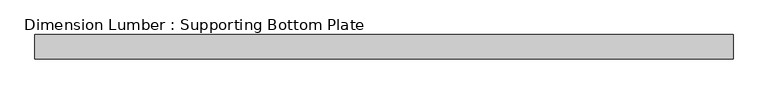
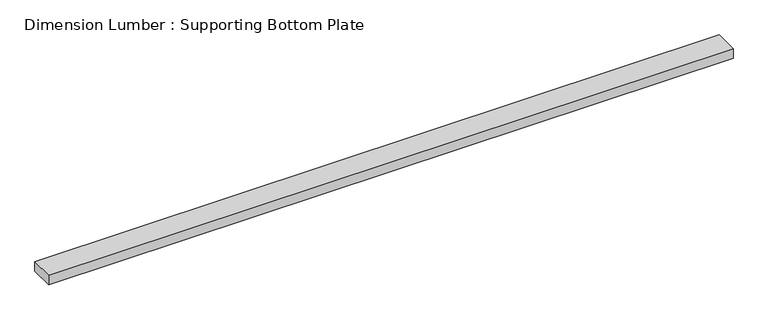
"""IFC4 building model written with IfcOpenShell, lengths in millimetres: beam geometry, Dimension Lumber : Supporting Bottom Plate."""

from ifc_helpers import new_model, si_unit, frame, origin, place, context, project, spatial, polyline, outline, extrude, source, transform, mapped, element, save


def dimension_lumber_supporting_bottom_plate_050ef5e1(model_context):
    return source(origin(), model_context, "Body", "SweptSolid", [
        extrude(outline(polyline([(1279.525, 44.45), (1279.525, -44.45), (-1279.525, -44.45), (-1279.525, 44.45), (1279.525, 44.45)])), frame((0.0, 0.0, -19.05), z_axis=(0.0, 0.0, 1.0), x_axis=(1.0, 0.0, 0.0)), (0.0, 0.0, 1.0), 38.1),
    ])


if __name__ == "__main__":
    model = new_model("IFC4")
    model_context = context("Model", 3, world=origin())
    ifc_project = project(units=[si_unit("LENGTHUNIT", "METRE", prefix="MILLI")], contexts=[model_context])
    site = spatial("IfcSite", under=ifc_project)
    building = spatial("IfcBuilding", under=site)
    placement = place(None, origin())
    dimension_lumber_supporting_bottom_plate_shape = dimension_lumber_supporting_bottom_plate_050ef5e1(model_context)
    element("IfcBeam", 1, ObjectType="Dimension Lumber : Supporting Bottom Plate", at=placement, inside=building, context=model_context, shape_type="MappedRepresentation", body=[
        mapped(dimension_lumber_supporting_bottom_plate_shape, transform((0.0, 0.0, 0.0), x_axis=(1.0, 0.0, 0.0), y_axis=(0.0, 1.0, 0.0), z_axis=(0.0, 0.0, 1.0))),
    ])
    save(model, "model.ifc")

# Revit data of these elements
# Type "Dimension Lumber : Supporting Bottom Plate"
#   Assembly Code = "B10"
#   A = 0.0364583 SF
#   Length [instance default] = 5' - 0"
#   b = 0' - 3 1/2"
#   d = 0' - 1 1/2"
#   Structural Material [instance default] = Softwood, Lumber
# Element 1 (IfcBeam, "Dimension Lumber : Supporting Bottom Plate")
#   Structural Material = Douglas Fir #2
#   Materials on its faces: "Douglas Fir #2"
# Materials
#   "Softwood, Lumber": class "Wood", colour RGB 223 192 134, transparency 0, Description = "Pinus Echinata", Cost = 0
#   "Douglas Fir #2": class "Wood", colour RGB 223 192 134, transparency 0, Description = "Pinus Echinata", Cost = 0
